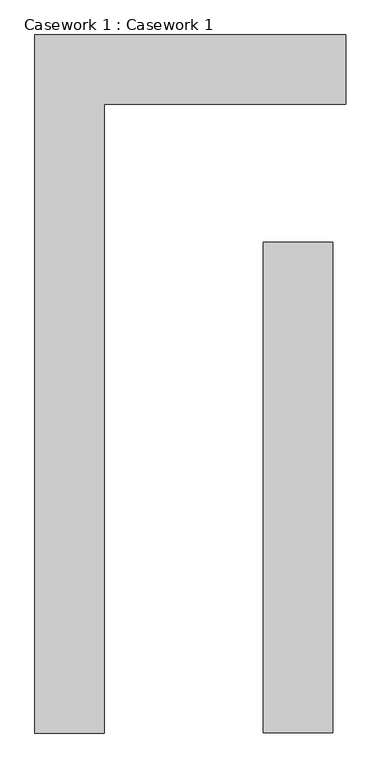
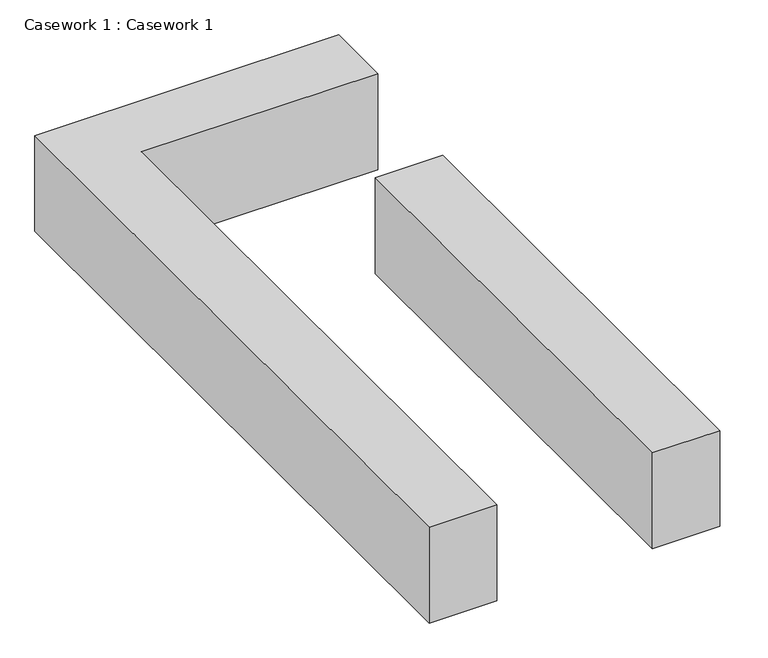
"""IFC4 building model written with IfcOpenShell, lengths in millimetres: furniture geometry, Casework 1 : Casework 1."""

from ifc_helpers import new_model, si_unit, origin, origin_with_axes, place, context, project, spatial, polyline, outline, extrude, source, transform, mapped, element, save


def casework_1_casework_1_d615d7ec(model_context):
    return source(origin(), model_context, "Body", "SweptSolid", [
        extrude(outline(polyline([(653847.1867239, -574091.7445091), (653847.1867239, -567932.6413841), (656590.3867239, -567932.6413841), (656590.3867239, -568542.2413841), (654456.7867239, -568542.2413841), (654456.7867239, -574091.7445091), (653847.1867239, -574091.7445091)])), origin_with_axes(), (0.0, 0.0, 1.0), 914.4),
        extrude(outline(polyline([(655863.3117239, -574088.9663841), (655863.3117239, -569761.4413841), (656472.9117239, -569761.4413841), (656472.9117239, -574088.9663841), (655863.3117239, -574088.9663841)])), origin_with_axes(), (0.0, 0.0, 1.0), 914.4),
    ])


if __name__ == "__main__":
    model = new_model("IFC4")
    model_context = context("Model", 3, world=origin())
    ifc_project = project(units=[si_unit("LENGTHUNIT", "METRE", prefix="MILLI")], contexts=[model_context])
    site = spatial("IfcSite", under=ifc_project)
    building = spatial("IfcBuilding", under=site)
    placement = place(None, origin())
    casework_1_casework_1_shape = casework_1_casework_1_d615d7ec(model_context)
    element("IfcFurniture", 1, ObjectType="Casework 1 : Casework 1", at=placement, inside=building, context=model_context, shape_type="MappedRepresentation", body=[
        mapped(casework_1_casework_1_shape, transform((0.0, 0.0, 0.0), x_axis=(1.0, 0.0, 0.0), y_axis=(0.0, 1.0, 0.0), z_axis=(0.0, 0.0, 1.0))),
    ])
    save(model, "model.ifc")
